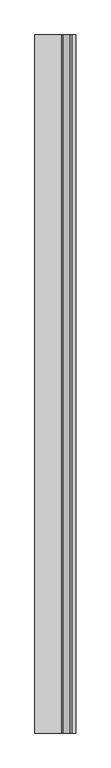
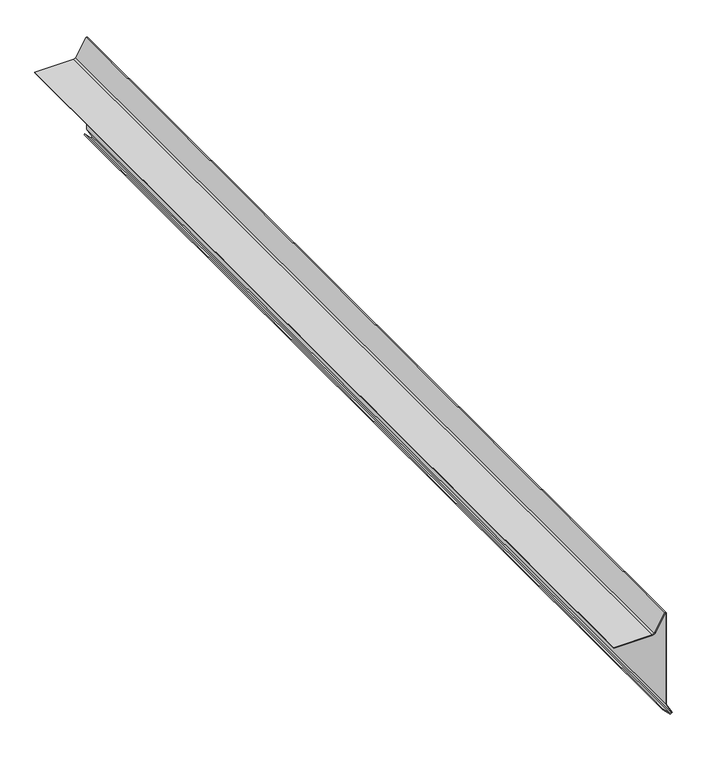
"""IFC4 building model written with IfcOpenShell, lengths in millimetres: proxy geometry, GRAVEL STOP005 3784 : GRAVEL STOP005 3784."""

from ifc_helpers import new_model, si_unit, frame, origin, place, context, project, spatial, polyline, outline, extrude, source, transform, mapped, element, save


def generic_models_bb7cdfd3(model_context):
    return source(origin(), model_context, "Body", "SweptSolid", [
        extrude(outline(polyline([(40077.410403, -4353.4420496), (40080.5182783, -4349.3681054), (40101.8558531, -4361.0170744), (40294.5307525, -4361.0170744), (40295.3431515, -4364.0489887), (40259.5408757, -4384.7194423), (40257.3744784, -4388.4717525), (40257.3744784, -4465.9296592), (40255.9633674, -4465.9296592), (40255.9633674, -4388.0936464), (40258.5078708, -4383.6864373), (40293.699878, -4363.3683225), (40293.447969, -4362.4281854), (40101.495749, -4362.4281854), (40080.9054201, -4351.1871656), (40079.2807815, -4353.3168157), (40092.8027062, -4366.8387404), (40091.8049, -4367.8365465), (40077.410403, -4353.4420496)])), frame((0.0, -1065.5906573, 0.0), z_axis=(0.0, 1.0, 0.0), x_axis=(0.0, 0.0, 1.0)), (0.0, 0.0, 1.0), 2000.25),
    ])


if __name__ == "__main__":
    model = new_model("IFC4")
    model_context = context("Model", 3, world=origin())
    ifc_project = project(units=[si_unit("LENGTHUNIT", "METRE", prefix="MILLI")], contexts=[model_context])
    site = spatial("IfcSite", under=ifc_project)
    building = spatial("IfcBuilding", under=site)
    placement = place(None, origin())
    generic_models_shape = generic_models_bb7cdfd3(model_context)
    element("IfcBuildingElementProxy", 1, Name="GRAVEL STOP005 3784 : GRAVEL STOP005 3784", ObjectType="GRAVEL STOP005 3784 : GRAVEL STOP005 3784", at=placement, inside=building, context=model_context, shape_type="MappedRepresentation", body=[
        mapped(generic_models_shape, transform((0.0, 0.0, 0.0), x_axis=(1.0, 0.0, 0.0), y_axis=(0.0, 1.0, 0.0), z_axis=(0.0, 0.0, 1.0))),
    ])
    save(model, "model.ifc")

# Revit data of these elements
# Type "GRAVEL STOP005 3784 : GRAVEL STOP005 3784"
#   NameOverride = "GRAVEL STOP005"
# Element 1 (IfcBuildingElementProxy, "GRAVEL STOP005 3784 : GRAVEL STOP005 3784")
#   Materials on its faces: "GRAVEL STOP REQUIRED WITH GRAVEL SURFACE SYSTEMS"
# Materials
#   "GRAVEL STOP REQUIRED WITH GRAVEL SURFACE SYSTEMS": class "Unassigned", colour RGB 170 170 127, transparency 0
